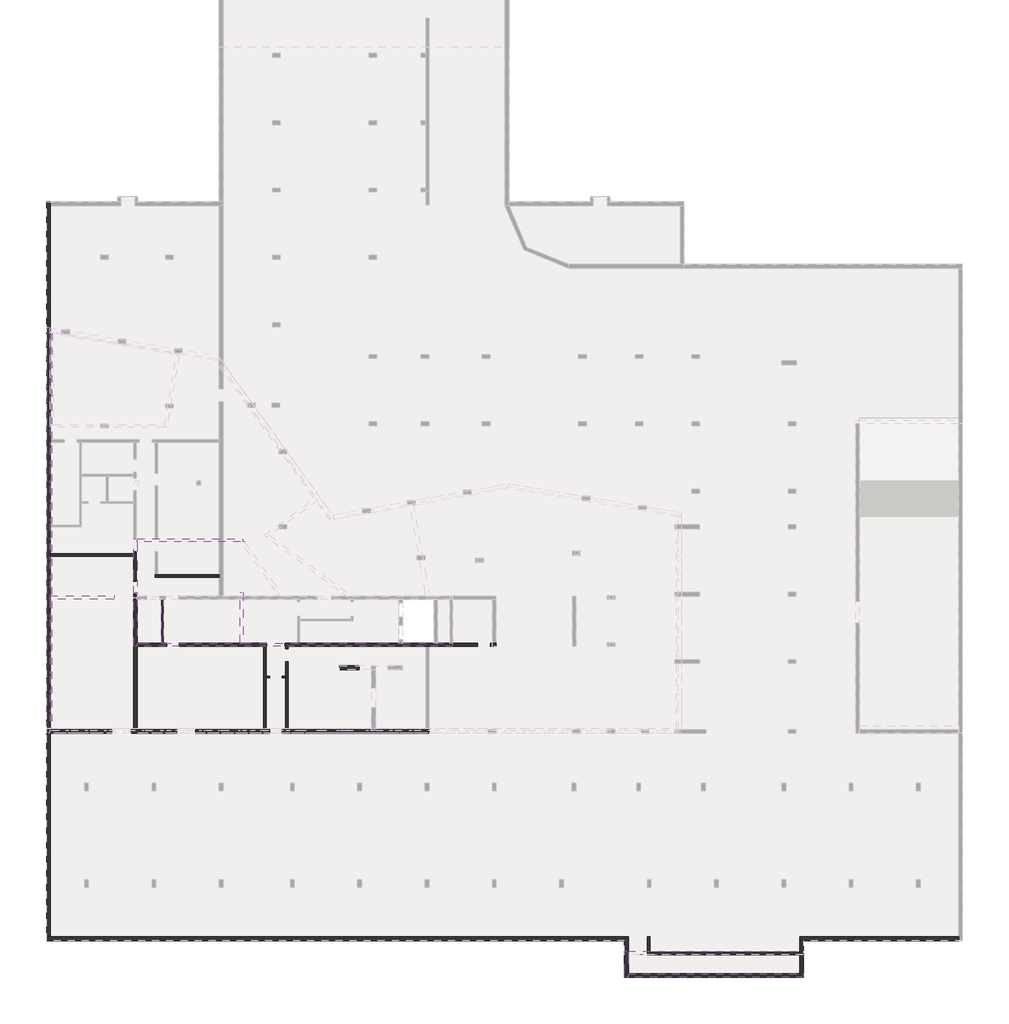
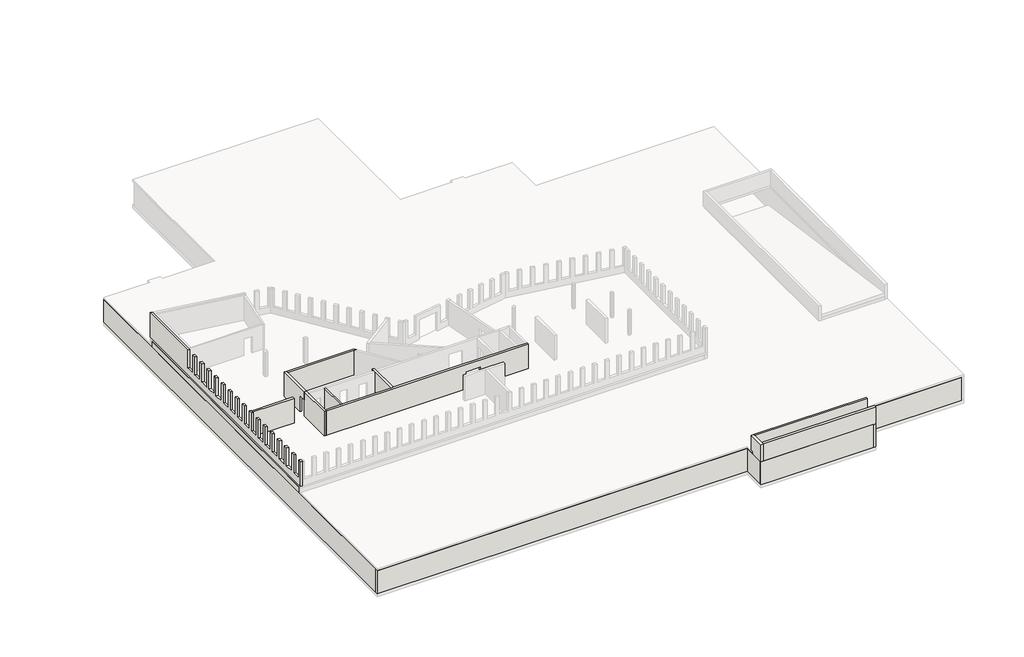
# One storey, part 1 of 4: 32 walls.
"""IFC4 building model written with IfcOpenShell, lengths in millimetres."""

from ifc_helpers import new_model, si_unit, frame, origin, place, context, project, spatial, polyline, outline, extrude, faceted_brep, element, save

model = new_model("IFC4")

# Units and contexts
model_context = context("Model", 3, world=origin())
ifc_project = project(units=[si_unit("LENGTHUNIT", "METRE", prefix="MILLI")], contexts=[model_context])

# Site, building, storey
site = spatial("IfcSite", under=ifc_project)
building = spatial("IfcBuilding", under=site)
storey = spatial("IfcBuildingStorey", under=building, Name="01_UG_OKFB_-4,20", Elevation=-4200.0)

# Walls
placement = place(None, origin())
element("IfcWall", 1, ObjectType="5dki Lochfassade 26cm C30/37", at=placement, inside=storey, context=model_context, shape_type="Brep", body=[
    faceted_brep([(130.0010047, 22777.9895381, 710.0), (130.0010047, 22777.9895381, 3060.0), (130.0010047, 22357.0124158, 3060.0), (130.0010047, 22357.0124158, 710.0), (130.0010047, 21277.0124158, 710.0), (130.0010047, 21277.0124158, 3060.0), (130.0010047, 20857.0124158, 3060.0), (130.0010047, 20857.0124158, 710.0), (130.0010047, 19777.0124158, 710.0), (130.0010047, 19777.0124158, 3060.0), (130.0010047, 19357.0124158, 3060.0), (130.0010047, 19357.0124158, 710.0), (130.0010047, 18277.0124158, 710.0), (130.0010047, 18277.0124158, 3060.0), (130.0010047, 17857.0124158, 3060.0), (130.0010047, 17857.0124158, 710.0), (130.0010047, 16777.0124158, 710.0), (130.0010047, 16777.0124158, 3060.0), (130.0010047, 16357.0124158, 3060.0), (130.0010047, 16357.0124158, 710.0), (130.0010047, 15277.0124158, 710.0), (130.0010047, 15277.0124158, 3060.0), (130.0010047, 14857.0124158, 3060.0), (130.0010047, 14857.0124158, 710.0), (130.0010047, 13777.0124158, 710.0), (130.0010047, 13777.0124158, 3060.0), (130.0010047, 13357.0124158, 3060.0), (130.0010047, 13357.0124158, 710.0), (130.0010047, 12277.0124158, 710.0), (130.0010047, 12277.0124158, 3060.0), (130.0010047, 11857.0124158, 3060.0), (130.0010047, 11857.0124158, 710.0), (130.0010047, 10777.0124158, 710.0), (130.0010047, 10777.0124158, 3060.0), (130.0010047, 10692.0124295, 3060.0), (130.0010047, 10442.0124295, 3060.0), (130.0010047, 10357.0124158, 3060.0), (130.0010047, 10357.0124158, 710.0), (130.0010047, 9277.0124158, 710.0), (130.0010047, 9277.0124158, 3060.0), (130.0010047, 8857.0124158, 3060.0), (130.0010047, 8857.0124158, 710.0), (130.0010047, 7777.0124158, 710.0), (130.0010047, 7777.0124158, 3060.0), (130.0010047, 7357.0124158, 3060.0), (130.0010047, 7357.0124158, 710.0), (130.0010047, 6277.0124158, 710.0), (130.0010047, 6277.0124158, 3060.0), (130.0010047, 5857.0124158, 3060.0), (130.0010047, 5857.0124158, 710.0), (130.0010047, 4777.0124158, 710.0), (130.0010047, 4777.0124158, 3060.0), (130.0010047, 4357.0124158, 3060.0), (130.0010047, 4357.0124158, 710.0), (130.0010047, 3277.0124158, 710.0), (130.0010047, 3277.0124158, 3060.0), (130.0010047, 2857.0124158, 3060.0), (130.0010047, 2857.0124158, 710.0), (130.0010047, 1777.0124158, 710.0), (130.0010047, 1777.0124158, 3060.0), (130.0010047, 1357.0124158, 3060.0), (130.0010047, 1357.0124158, 710.0), (130.0010047, 277.0124158, 710.0), (130.0010047, 277.0124158, 3060.0), (130.0010047, 130.000972, 3060.0), (130.0010047, -129.999028, 3060.0), (130.0010047, -129.999028, -150.0), (130.0010047, 130.000972, -150.0), (130.0010047, 10442.0124295, -150.0), (130.0010047, 10692.0124295, -150.0), (130.0010047, 31548.6978518, -150.0), (130.0010047, 31812.2980067, -150.0), (130.0010047, 31812.2980067, 3060.0), (130.0010047, 31548.6978518, 3060.0), (130.0010047, 23857.9895381, 3060.0), (130.0010047, 23857.9895381, 710.0), (-129.9989953, 22357.0124158, 3060.0), (-129.9989953, 22777.9895381, 3060.0), (-129.9989953, 22777.9895381, 710.0), (-129.9989953, 23857.9895381, 710.0), (-129.9989953, 23857.9895381, 3060.0), (-129.9989953, 31855.7150729, 3060.0), (-129.9989953, 31855.7150729, -150.0), (-129.9989953, -129.9990284, -150.0), (-129.9989953, -129.9990284, 3060.0), (-129.9989953, 277.0124158, 3060.0), (-129.9989953, 277.0124158, 710.0), (-129.9989953, 1357.0124158, 710.0), (-129.9989953, 1357.0124158, 3060.0), (-129.9989953, 1777.0124158, 3060.0), (-129.9989953, 1777.0124158, 710.0), (-129.9989953, 2857.0124158, 710.0), (-129.9989953, 2857.0124158, 3060.0), (-129.9989953, 3277.0124158, 3060.0), (-129.9989953, 3277.0124158, 710.0), (-129.9989953, 4357.0124158, 710.0), (-129.9989953, 4357.0124158, 3060.0), (-129.9989953, 4777.0124158, 3060.0), (-129.9989953, 4777.0124158, 710.0), (-129.9989953, 5857.0124158, 710.0), (-129.9989953, 5857.0124158, 3060.0), (-129.9989953, 6277.0124158, 3060.0), (-129.9989953, 6277.0124158, 710.0), (-129.9989953, 7357.0124158, 710.0), (-129.9989953, 7357.0124158, 3060.0), (-129.9989953, 7777.0124158, 3060.0), (-129.9989953, 7777.0124158, 710.0), (-129.9989953, 8857.0124158, 710.0), (-129.9989953, 8857.0124158, 3060.0), (-129.9989953, 9277.0124158, 3060.0), (-129.9989953, 9277.0124158, 710.0), (-129.9989953, 10357.0124158, 710.0), (-129.9989953, 10357.0124158, 3060.0), (-129.9989953, 10777.0124158, 3060.0), (-129.9989953, 10777.0124158, 710.0), (-129.9989953, 11857.0124158, 710.0), (-129.9989953, 11857.0124158, 3060.0), (-129.9989953, 12277.0124158, 3060.0), (-129.9989953, 12277.0124158, 710.0), (-129.9989953, 13357.0124158, 710.0), (-129.9989953, 13357.0124158, 3060.0), (-129.9989953, 13777.0124158, 3060.0), (-129.9989953, 13777.0124158, 710.0), (-129.9989953, 14857.0124158, 710.0), (-129.9989953, 14857.0124158, 3060.0), (-129.9989953, 15277.0124158, 3060.0), (-129.9989953, 15277.0124158, 710.0), (-129.9989953, 16357.0124158, 710.0), (-129.9989953, 16357.0124158, 3060.0), (-129.9989953, 16777.0124158, 3060.0), (-129.9989953, 16777.0124158, 710.0), (-129.9989953, 17857.0124158, 710.0), (-129.9989953, 17857.0124158, 3060.0), (-129.9989953, 18277.0124158, 3060.0), (-129.9989953, 18277.0124158, 710.0), (-129.9989953, 19357.0124158, 710.0), (-129.9989953, 19357.0124158, 3060.0), (-129.9989953, 19777.0124158, 3060.0), (-129.9989953, 19777.0124158, 710.0), (-129.9989953, 20857.0124158, 710.0), (-129.9989953, 20857.0124158, 3060.0), (-129.9989953, 21277.0124158, 3060.0), (-129.9989953, 21277.0124158, 710.0), (-129.9989953, 22357.0124158, 710.0)], [[[0, 1, 2, 3, 4, 5, 6, 7, 8, 9, 10, 11, 12, 13, 14, 15, 16, 17, 18, 19, 20, 21, 22, 23, 24, 25, 26, 27, 28, 29, 30, 31, 32, 33, 34, 35, 36, 37, 38, 39, 40, 41, 42, 43, 44, 45, 46, 47, 48, 49, 50, 51, 52, 53, 54, 55, 56, 57, 58, 59, 60, 61, 62, 63, 64, 65, 66, 67, 68, 69, 70, 71, 72, 73, 74, 75]], [[76, 77, 78, 79, 80, 81, 82, 83, 84, 85, 86, 87, 88, 89, 90, 91, 92, 93, 94, 95, 96, 97, 98, 99, 100, 101, 102, 103, 104, 105, 106, 107, 108, 109, 110, 111, 112, 113, 114, 115, 116, 117, 118, 119, 120, 121, 122, 123, 124, 125, 126, 127, 128, 129, 130, 131, 132, 133, 134, 135, 136, 137, 138, 139, 140, 141, 142, 143]], [[71, 70, 69, 68, 67, 66, 83, 82]], [[84, 65, 64, 63, 85]], [[60, 59, 89, 88]], [[56, 55, 93, 92]], [[52, 51, 97, 96]], [[48, 47, 101, 100]], [[44, 43, 105, 104]], [[40, 39, 109, 108]], [[36, 35, 34, 33, 113, 112]], [[30, 29, 117, 116]], [[26, 25, 121, 120]], [[22, 21, 125, 124]], [[18, 17, 129, 128]], [[14, 13, 133, 132]], [[10, 9, 137, 136]], [[6, 5, 141, 140]], [[2, 1, 77, 76]], [[74, 73, 72, 81, 80]], [[72, 71, 82, 81]], [[66, 65, 84, 83]], [[87, 61, 60, 88]], [[62, 86, 85, 63]], [[61, 87, 86, 62]], [[92, 91, 57, 56]], [[90, 89, 59, 58]], [[91, 90, 58, 57]], [[96, 95, 53, 52]], [[94, 93, 55, 54]], [[95, 94, 54, 53]], [[100, 99, 49, 48]], [[98, 97, 51, 50]], [[99, 98, 50, 49]], [[104, 103, 45, 44]], [[102, 101, 47, 46]], [[103, 102, 46, 45]], [[108, 107, 41, 40]], [[106, 105, 43, 42]], [[107, 106, 42, 41]], [[112, 111, 37, 36]], [[110, 109, 39, 38]], [[111, 110, 38, 37]], [[116, 115, 31, 30]], [[114, 113, 33, 32]], [[115, 114, 32, 31]], [[120, 119, 27, 26]], [[118, 117, 29, 28]], [[119, 118, 28, 27]], [[124, 123, 23, 22]], [[122, 121, 25, 24]], [[123, 122, 24, 23]], [[128, 127, 19, 18]], [[126, 125, 21, 20]], [[127, 126, 20, 19]], [[132, 131, 15, 14]], [[130, 129, 17, 16]], [[131, 130, 16, 15]], [[136, 135, 11, 10]], [[134, 133, 13, 12]], [[135, 134, 12, 11]], [[140, 139, 7, 6]], [[138, 137, 9, 8]], [[139, 138, 8, 7]], [[76, 143, 3, 2]], [[142, 141, 5, 4]], [[143, 142, 4, 3]], [[80, 79, 75, 74]], [[78, 77, 1, 0]], [[79, 78, 0, 75]]]),
])
element("IfcWall", 2, ObjectType="5dki STB-Wand Kern 25cm C30/37", at=placement, inside=storey, context=model_context, shape_type="Brep", body=[
    faceted_brep([(6989.9999766, 15192.0124447, 3060.0), (6989.9999766, 14942.0124447, 3060.0), (6989.9999766, 10947.0136187, 3060.0), (6989.9999766, 10947.0136187, 1985.0), (6989.9999766, 11957.013616, 1985.0), (6989.9999766, 11957.013616, -150.0), (6989.9999766, 14942.0124447, -150.0), (6989.9999766, 15192.0124447, -150.0), (6739.9999766, 10947.0136187, 3060.0), (6739.9999766, 15192.0124447, 3060.0), (6739.9999766, 15192.0124447, -150.0), (6739.9999766, 11957.013616, -150.0), (6739.9999766, 11957.013616, 1985.0), (6739.9999766, 10947.0136187, 1985.0)], [[[0, 1, 2, 3, 4, 5, 6, 7]], [[8, 9, 10, 11, 12, 13]], [[10, 7, 6, 5, 11]], [[2, 1, 0, 9, 8]], [[2, 8, 13, 3]], [[0, 7, 10, 9]], [[4, 12, 11, 5]], [[12, 4, 3, 13]]]),
])
element("IfcWall", 3, ObjectType="5dki STB-Wand Kern 25cm C30/37", at=placement, inside=storey, context=model_context, shape_type="Brep", body=[
    faceted_brep([(6989.9999766, 14942.0124447, -150.0), (15141.8279932, 14942.0124447, -150.0), (15449.8792779, 14942.0124447, -150.0), (15449.8792779, 14942.0124447, 3060.0), (15141.8279932, 14942.0124447, 3060.0), (6989.9999766, 14942.0124447, 3060.0), (6989.9999766, 15192.0124447, -150.0), (6989.9999766, 15192.0124447, 3060.0), (15269.8915173, 15192.0124447, 3060.0), (15269.8915173, 15192.0124447, -150.0)], [[[0, 1, 2, 3, 4, 5]], [[6, 7, 8, 9]], [[2, 1, 0, 6, 9]], [[5, 4, 3, 8, 7]], [[0, 5, 7, 6]], [[3, 2, 9, 8]]]),
])
element("IfcWall", 4, ObjectType="5dki STB-Wand Kern 25cm C30/37", at=placement, inside=storey, context=model_context, shape_type="Brep", body=[
    faceted_brep([(6739.9995723, 10947.0136187, -150.0), (6739.9995723, 6740.0000204, -150.0), (6739.9995723, 6740.0000204, 3060.0), (6739.9995723, 10947.0136187, 3060.0), (6739.9995723, 10947.0136187, 1985.0), (6989.9995723, 10947.0136187, -150.0), (6989.9995723, 10947.0136187, 1985.0), (6989.9995723, 10947.0136187, 3060.0), (6989.9995723, 10662.0127052, 3060.0), (6989.9995723, 10442.0127052, 3060.0), (6989.9995723, 6960.0000208, 3060.0), (6989.9995723, 6740.0000208, 3060.0), (6989.9995723, 6740.0000208, -150.0), (6989.9995723, 6960.0000208, -150.0), (6989.9995723, 10442.0127052, -150.0), (6989.9995723, 10662.0127052, -150.0)], [[[0, 1, 2, 3, 4]], [[5, 6, 7, 8, 9, 10, 11, 12, 13, 14, 15]], [[1, 0, 5, 15, 14, 13, 12]], [[3, 2, 11, 10, 9, 8, 7]], [[0, 4, 3, 7, 6, 5]], [[2, 1, 12, 11]]]),
])
element("IfcWall", 5, ObjectType="5dki STB-Wand Kern 22cm C30/37", at=placement, inside=storey, context=model_context, shape_type="Brep", body=[
    faceted_brep([(31841.999935, 6740.0000516, 3060.0), (6989.9995723, 6740.0000208, 3060.0), (6989.9995723, 6740.0000208, -150.0), (24166.9999591, 6740.0000421, -150.0), (24166.999888, 6740.0000421, 2110.0), (25926.9999591, 6740.0000443, 2110.0), (25927.000338, 6740.0000443, -150.0), (31841.999935, 6740.0000516, -150.0), (6989.9995723, 6960.0000208, 3060.0), (8916.9999886, 6960.0000232, 3060.0), (9066.9999886, 6960.0000233, 3060.0), (15117.0008797, 6960.0000309, 3060.0), (15367.0008797, 6960.0000312, 3060.0), (27641.9999886, 6960.0000464, 3060.0), (27891.9999886, 6960.0000467, 3060.0), (30391.9999891, 6960.0000498, 3060.0), (30641.9999891, 6960.0000501, 3060.0), (31641.9999382, 6960.0000514, 3060.0), (31841.9999382, 6960.0000516, 3060.0), (31841.9999382, 6960.0000516, -150.0), (31641.9999382, 6960.0000514, -150.0), (30641.9999891, 6960.0000501, -150.0), (30391.9999891, 6960.0000498, -150.0), (27891.9999886, 6960.0000467, -150.0), (27641.9999886, 6960.0000464, -150.0), (25926.9999588, 6960.0000443, -150.0), (25927.000338, 6960.0000443, 2110.0), (24166.9999588, 6960.0000421, 2110.0), (24166.999888, 6960.0000421, -150.0), (15367.0008797, 6960.0000312, -150.0), (15117.0008797, 6960.0000309, -150.0), (9066.9999886, 6960.0000233, -150.0), (8916.9999886, 6960.0000232, -150.0), (6989.9995723, 6960.0000208, -150.0)], [[[0, 1, 2, 3, 4, 5, 6, 7]], [[8, 9, 10, 11, 12, 13, 14, 15, 16, 17, 18, 19, 20, 21, 22, 23, 24, 25, 26, 27, 28, 29, 30, 31, 32, 33]], [[2, 33, 32, 31, 30, 29, 28, 3]], [[19, 7, 6, 25, 24, 23, 22, 21, 20]], [[1, 0, 18, 17, 16, 15, 14, 13, 12, 11, 10, 9, 8]], [[2, 1, 8, 33]], [[0, 7, 19, 18]], [[5, 26, 25, 6]], [[26, 5, 4, 27]], [[27, 4, 3, 28]]]),
])
element("IfcWall", 6, ObjectType="5dki STB-Wand Kern 25cm C30/37", at=placement, inside=storey, context=model_context, shape_type="SweptSolid", body=[
    extrude(outline(polyline([(15117.0008797, 6960.0000309), (15117.0008797, 10990.000031), (15367.0008797, 10990.000031), (15367.0008797, 6960.0000312), (15117.0008797, 6960.0000309)])), frame((0.0, 0.0, -150.0), z_axis=(0.0, 0.0, 1.0), x_axis=(1.0, 0.0, 0.0)), (0.0, 0.0, 1.0), 3210.0),
])
element("IfcWall", 7, ObjectType="5dki STB-Wand Kern 15cm C30/37", at=placement, inside=storey, context=model_context, shape_type="SweptSolid", body=[
    extrude(outline(polyline([(8916.9999886, 6960.0000232), (8916.9999886, 10442.0127087), (9066.9999886, 10442.0127089), (9066.9999886, 6960.0000233), (8916.9999886, 6960.0000232)])), frame((0.0, 0.0, -150.0), z_axis=(0.0, 0.0, 1.0), x_axis=(1.0, 0.0, 0.0)), (0.0, 0.0, 1.0), 3210.0),
])
element("IfcWall", 8, ObjectType="5dki STB-Wand Kern 22cm C30/37", at=placement, inside=storey, context=model_context, shape_type="Brep", body=[
    faceted_brep([(35269.999309, 6740.0016809, -1200.0), (29969.9992095, 6740.0014024, -1200.0), (29769.9992095, 6740.0013919, -1200.0), (18876.9410665, 6740.0008196, -1200.0), (18676.9410665, 6740.0008091, -1200.0), (17176.9410653, 6740.0007303, -1200.0), (16976.9410653, 6740.0007198, -1200.0), (6990.0006232, 6740.0001951, -1200.0), (6740.000624, 6740.0001819, -1200.0), (6740.000624, 6740.0001819, -4200.0), (6990.0006232, 6740.0001951, -4200.0), (9318.2481994, 6740.0003174, -4200.0), (9318.2482224, 6740.0003174, -2065.0), (10328.2481994, 6740.0003705, -2065.0), (10328.248215, 6740.0003705, -4200.0), (16976.9410653, 6740.0007198, -4200.0), (17176.9410653, 6740.0007303, -4200.0), (17186.9410653, 6740.0007308, -4200.0), (17186.9410832, 6740.0007308, -2065.0), (18666.9410653, 6740.0008086, -2065.0), (18666.9410837, 6740.0008086, -4200.0), (18676.9410665, 6740.0008091, -4200.0), (18876.9410665, 6740.0008196, -4200.0), (29769.9992095, 6740.0013919, -4200.0), (29969.9992095, 6740.0014024, -4200.0), (33806.9997689, 6740.001604, -4200.0), (33806.9997878, 6740.001604, -2065.0), (34816.9997689, 6740.0016571, -2065.0), (34816.9998011, 6740.0016571, -4200.0), (35269.999309, 6740.0016809, -4200.0), (6740.0006072, 6960.0001819, -1200.0), (6990.0006072, 6960.0001951, -1200.0), (8916.9991145, 6960.0002963, -1200.0), (9066.9991145, 6960.0003042, -1200.0), (19626.9996762, 6960.000859, -1200.0), (19776.9996762, 6960.0008669, -1200.0), (27642.0002944, 6960.0012801, -1200.0), (27892.0002944, 6960.0012933, -1200.0), (30391.9991141, 6960.0014246, -1200.0), (30641.9991141, 6960.0014377, -1200.0), (31641.9991143, 6960.0014903, -1200.0), (31841.9991143, 6960.0015008, -1200.0), (34969.9993085, 6960.0016651, -1200.0), (35269.9993085, 6960.0016809, -1200.0), (35269.9993085, 6960.0016809, -4200.0), (34969.9993085, 6960.0016651, -4200.0), (34816.9997573, 6960.0016571, -4200.0), (34816.9997599, 6960.0016571, -2065.0), (33806.9997573, 6960.001604, -2065.0), (33806.9997466, 6960.001604, -4200.0), (31841.9991143, 6960.0015008, -4200.0), (31641.9991143, 6960.0014903, -4200.0), (30641.9991141, 6960.0014377, -4200.0), (30391.9991141, 6960.0014246, -4200.0), (27892.0002944, 6960.0012933, -4200.0), (27642.0002944, 6960.0012801, -4200.0), (19776.9996762, 6960.0008669, -4200.0), (19626.9996762, 6960.000859, -4200.0), (18666.9410538, 6960.0008086, -4200.0), (18666.9410424, 6960.0008086, -2065.0), (17186.9410538, 6960.0007308, -2065.0), (17186.941042, 6960.0007308, -4200.0), (10328.2481878, 6960.0003705, -4200.0), (10328.2481738, 6960.0003705, -2065.0), (9318.2481878, 6960.0003174, -2065.0), (9318.2481812, 6960.0003174, -4200.0), (9066.9991145, 6960.0003042, -4200.0), (8916.9991145, 6960.0002963, -4200.0), (6990.0006072, 6960.0001951, -4200.0), (6740.0006072, 6960.0001819, -4200.0)], [[[0, 1, 2, 3, 4, 5, 6, 7, 8, 9, 10, 11, 12, 13, 14, 15, 16, 17, 18, 19, 20, 21, 22, 23, 24, 25, 26, 27, 28, 29]], [[30, 31, 32, 33, 34, 35, 36, 37, 38, 39, 40, 41, 42, 43, 44, 45, 46, 47, 48, 49, 50, 51, 52, 53, 54, 55, 56, 57, 58, 59, 60, 61, 62, 63, 64, 65, 66, 67, 68, 69]], [[44, 29, 28, 46, 45]], [[9, 69, 68, 67, 66, 65, 11, 10]], [[49, 25, 24, 23, 22, 21, 20, 58, 57, 56, 55, 54, 53, 52, 51, 50]], [[14, 62, 61, 17, 16, 15]], [[8, 7, 6, 5, 4, 3, 2, 1, 0, 43, 42, 41, 40, 39, 38, 37, 36, 35, 34, 33, 32, 31, 30]], [[0, 29, 44, 43]], [[9, 8, 30, 69]], [[27, 47, 46, 28]], [[47, 27, 26, 48]], [[48, 26, 25, 49]], [[64, 12, 11, 65]], [[12, 64, 63, 13]], [[13, 63, 62, 14]], [[60, 18, 17, 61]], [[18, 60, 59, 19]], [[19, 59, 58, 20]]]),
])
element("IfcWall", 9, ObjectType="5dki STB-Wand Kern 25cm C30/37", at=placement, inside=storey, context=model_context, shape_type="SweptSolid", body=[
    extrude(outline(polyline([(6740.0006072, 6960.0001819), (6740.0003427, 10442.0129553), (6990.0003427, 10442.0129495), (6990.0006072, 6960.0001951), (6740.0006072, 6960.0001819)])), frame((0.0, 0.0, -4200.0), z_axis=(0.0, 0.0, 1.0), x_axis=(1.0, 0.0, 0.0)), (0.0, 0.0, 1.0), 3000.0),
])
element("IfcWall", 10, ObjectType="5dki STB-Wand Kern 15cm C30/37", at=placement, inside=storey, context=model_context, shape_type="SweptSolid", body=[
    extrude(outline(polyline([(8916.9991145, 6960.0002963), (8916.9991145, 10442.012905), (9066.9991145, 10442.0129015), (9066.9991145, 6960.0003042), (8916.9991145, 6960.0002963)])), frame((0.0, 0.0, -4200.0), z_axis=(0.0, 0.0, 1.0), x_axis=(1.0, 0.0, 0.0)), (0.0, 0.0, 1.0), 3000.0),
])
element("IfcWall", 11, ObjectType="5dki STB-Wand 30cm WU C35/45", at=placement, inside=storey, context=model_context, shape_type="Brep", body=[
    faceted_brep([(71679.9986191, -16130.0005666, -4200.0), (59176.9101139, -16130.0005666, -4200.0), (59176.9101139, -16130.0005666, -1200.0), (71679.9986191, -16130.0005666, -1200.0), (71679.9986133, -16430.0005666, -4200.0), (71679.9986133, -16430.0005666, -1200.0), (59476.9101139, -16430.0005666, -1200.0), (59176.9101139, -16430.0005666, -1200.0), (59176.9101139, -16430.0005666, -4200.0), (59476.9101139, -16430.0005666, -4200.0)], [[[0, 1, 2, 3]], [[4, 5, 6, 7, 8, 9]], [[1, 0, 4, 9, 8]], [[3, 2, 7, 6, 5]], [[0, 3, 5, 4]], [[2, 1, 8, 7]]]),
])
element("IfcWall", 12, ObjectType="5dki STB-Wand 30cm WU C35/45", at=placement, inside=storey, context=model_context, shape_type="Brep", body=[
    faceted_brep([(59176.9101139, -16430.0005666, -4200.0), (59176.9101139, -17332.4969559, -4200.0), (59176.9101139, -17532.4969604, -4200.0), (59176.9101139, -19032.4966002, -4200.0), (59176.9101139, -19332.4966002, -4200.0), (59176.9101139, -19332.4966002, -1200.0), (59176.9101139, -19032.4966002, -1200.0), (59176.9101139, -17532.4969604, -1200.0), (59176.9101139, -17332.4969559, -1200.0), (59176.9101139, -16430.0005666, -1200.0), (59476.9101139, -16430.0005666, -4200.0), (59476.9101139, -16430.0005666, -1200.0), (59476.9101139, -19332.4966002, -1200.0), (59476.9101139, -19332.4966002, -4200.0)], [[[0, 1, 2, 3, 4, 5, 6, 7, 8, 9]], [[10, 11, 12, 13]], [[4, 3, 2, 1, 0, 10, 13]], [[9, 8, 7, 6, 5, 12, 11]], [[0, 9, 11, 10]], [[5, 4, 13, 12]]]),
])
element("IfcWall", 13, ObjectType="5dki STB-Wand 30cm WU C35/45", at=placement, inside=storey, context=model_context, shape_type="Brep", body=[
    faceted_brep([(59176.9101139, -19032.4966002, -4200.0), (45670.0209209, -19032.4966002, -4200.0), (45370.0209209, -19032.4966002, -4200.0), (45370.0209209, -19032.4966002, -1200.0), (45670.0209209, -19032.4966002, -1200.0), (59176.9101139, -19032.4966002, -1200.0), (59176.9101139, -19332.4966002, -4200.0), (59176.9101139, -19332.4966002, -1200.0), (45370.0209209, -19332.4966002, -1200.0), (45370.0209209, -19332.4966002, -4200.0)], [[[0, 1, 2, 3, 4, 5]], [[6, 7, 8, 9]], [[2, 1, 0, 6, 9]], [[5, 4, 3, 8, 7]], [[0, 5, 7, 6]], [[3, 2, 9, 8]]]),
])
element("IfcWall", 14, ObjectType="5dki STB-Wand 30cm WU C35/45", at=placement, inside=storey, context=model_context, shape_type="Brep", body=[
    faceted_brep([(45670.0209209, -19032.4966002, -4200.0), (45670.0209209, -16129.9998873, -4200.0), (45670.0209209, -16129.9998873, -1200.0), (45670.0209209, -19032.4966002, -1200.0), (45370.0209209, -19032.4966002, -4200.0), (45370.0209209, -19032.4966002, -1200.0), (45370.0209209, -16429.9998873, -1200.0), (45370.0209209, -16129.9998873, -1200.0), (45370.0209209, -16129.9998873, -4200.0), (45370.0209209, -16429.9998873, -4200.0)], [[[0, 1, 2, 3]], [[4, 5, 6, 7, 8, 9]], [[1, 0, 4, 9, 8]], [[3, 2, 7, 6, 5]], [[0, 3, 5, 4]], [[2, 1, 8, 7]]]),
])
element("IfcWall", 15, ObjectType="5dki STB-Wand 30cm WU C35/45", at=placement, inside=storey, context=model_context, shape_type="Brep", body=[
    faceted_brep([(45370.0209209, -16129.9998873, -4200.0), (169.9998112, -16129.9998873, -4200.0), (-130.0001888, -16129.9998873, -4200.0), (-130.0001888, -16129.9998873, -1200.0), (169.9998112, -16129.9998873, -1200.0), (45370.0209209, -16129.9998873, -1200.0), (45370.0209209, -16429.9998873, -4200.0), (45370.0209209, -16429.9998873, -1200.0), (-130.0001888, -16429.9998873, -1200.0), (-130.0001888, -16429.9998873, -4200.0)], [[[0, 1, 2, 3, 4, 5]], [[6, 7, 8, 9]], [[2, 1, 0, 6, 9]], [[5, 4, 3, 8, 7]], [[0, 5, 7, 6]], [[3, 2, 9, 8]]]),
])
element("IfcWall", 16, ObjectType="5dki STB-Wand 30cm WU C35/45", at=placement, inside=storey, context=model_context, shape_type="Brep", body=[
    faceted_brep([(169.9998112, -16129.9998873, -4200.0), (169.9998112, -129.9999484, -4200.0), (169.9998112, 170.0000516, -4200.0), (169.9998112, 13818.6536257, -4200.0), (169.9998112, 14018.6536257, -4200.0), (169.9998112, 22769.9814538, -4200.0), (169.9998112, 22969.9814538, -4200.0), (169.9998112, 41417.0011496, -4200.0), (169.9998112, 41717.0011496, -4200.0), (169.9998112, 41717.0011496, -1200.0), (169.9998112, 41417.0011496, -1200.0), (169.9998112, 22969.9814538, -1200.0), (169.9998112, 22769.9814538, -1200.0), (169.9998112, 14018.6536257, -1200.0), (169.9998112, 13818.6536257, -1200.0), (169.9998112, 170.0000516, -1200.0), (169.9998112, -129.9999484, -1200.0), (169.9998112, -16129.9998873, -1200.0), (-130.0001888, -16129.9998873, -4200.0), (-130.0001888, -16129.9998873, -1200.0), (-130.0001888, 41717.0011496, -1200.0), (-130.0001888, 41717.0011496, -4200.0)], [[[0, 1, 2, 3, 4, 5, 6, 7, 8, 9, 10, 11, 12, 13, 14, 15, 16, 17]], [[18, 19, 20, 21]], [[8, 7, 6, 5, 4, 3, 2, 1, 0, 18, 21]], [[17, 16, 15, 14, 13, 12, 11, 10, 9, 20, 19]], [[0, 17, 19, 18]], [[9, 8, 21, 20]]]),
])
element("IfcWall", 17, ObjectType="5dki Überzug 40cm C30/37", at=placement, inside=storey, context=model_context, shape_type="Brep", body=[
    faceted_brep([(269.9998112, 270.0010491, -1200.0), (269.9998112, 31383.3810859, -1200.0), (269.9998112, 31383.3810859, -400.0), (269.9998112, 270.0010491, -400.0), (-130.0001888, 270.0010491, -1200.0), (-130.0001888, 270.0010491, -950.0), (-130.0001888, 270.0010491, -400.0), (-130.0001888, 31450.1765724, -400.0), (-130.0001888, 31450.1765724, -950.0), (-130.0001888, 31450.1765724, -1200.0)], [[[0, 1, 2, 3]], [[4, 5, 6, 7, 8, 9]], [[1, 0, 4, 9]], [[3, 2, 7, 6]], [[2, 1, 9, 8, 7]], [[0, 3, 6, 5, 4]]]),
])
element("IfcWall", 18, ObjectType="5dki STB-Wand 12,5cm C20/25", at=placement, inside=storey, context=model_context, shape_type="Brep", body=[
    faceted_brep([(18676.94108, 4233.966015, -1200.0), (17176.9410795, 4233.9660069, -1200.0), (17176.9410795, 4233.9660069, -4200.0), (17421.9417385, 4233.9660083, -4200.0), (17421.9417453, 4233.9660083, -2065.0), (18431.9417385, 4233.9660137, -2065.0), (18431.9417669, 4233.9660137, -4200.0), (18676.94108, 4233.966015, -4200.0), (17176.9410788, 4358.9660069, -1200.0), (18676.9410794, 4358.966015, -1200.0), (18676.9410794, 4358.966015, -4200.0), (18431.9417378, 4358.9660137, -4200.0), (18431.9417669, 4358.9660137, -2065.0), (17421.9417378, 4358.9660083, -2065.0), (17421.9417453, 4358.9660083, -4200.0), (17176.9410788, 4358.9660069, -4200.0)], [[[0, 1, 2, 3, 4, 5, 6, 7]], [[8, 9, 10, 11, 12, 13, 14, 15]], [[2, 15, 14, 3]], [[10, 7, 6, 11]], [[1, 0, 9, 8]], [[2, 1, 8, 15]], [[0, 7, 10, 9]], [[5, 12, 11, 6]], [[12, 5, 4, 13]], [[13, 4, 3, 14]]]),
])
element("IfcWall", 19, ObjectType="5dki STB-Wand 20cm C25/30", at=placement, inside=storey, context=model_context, shape_type="Brep", body=[
    faceted_brep([(13469.9992636, 12367.0009111, -4200.0), (8640.0000033, 12367.0009111, -4200.0), (8440.0000033, 12367.0009111, -4200.0), (8440.0000033, 12367.0009111, -1200.0), (8640.0000033, 12367.0009111, -1200.0), (13469.9992636, 12367.0009111, -1200.0), (13469.9992584, 12167.0009111, -4200.0), (13469.9992584, 12167.0009111, -1200.0), (8439.9999991, 12167.0009111, -1200.0), (8439.9999991, 12167.0009111, -4200.0)], [[[0, 1, 2, 3, 4, 5]], [[6, 7, 8, 9]], [[2, 1, 0, 6, 9]], [[5, 4, 3, 8, 7]], [[0, 5, 7, 6]], [[3, 2, 9, 8]]]),
])
element("IfcWall", 20, ObjectType="5dki STB-Wand 20cm C30/37", at=placement, inside=storey, context=model_context, shape_type="Brep", body=[
    faceted_brep([(47169.9986162, -16129.9999339, -4200.0), (47169.9986162, -17529.9576362, -4200.0), (47169.9986162, -17529.9576362, -1200.0), (47169.9986162, -16129.9999339, -1200.0), (47369.9986162, -16129.9999339, -4200.0), (47369.9986162, -16129.9999339, -1200.0), (47369.9986162, -17329.9999295, -1200.0), (47369.9986162, -17529.9999339, -1200.0), (47369.9986162, -17529.9999339, -4200.0), (47369.9986162, -17329.9999295, -4200.0)], [[[0, 1, 2, 3]], [[4, 5, 6, 7, 8, 9]], [[1, 0, 4, 9, 8]], [[3, 2, 7, 6, 5]], [[0, 3, 5, 4]], [[2, 1, 8, 7]]]),
])
element("IfcWall", 21, ObjectType="5dki STB-Wand 20cm C30/37", at=placement, inside=storey, context=model_context, shape_type="SweptSolid", body=[
    extrude(outline(polyline([(59176.9101139, -17532.4969604), (47369.9986162, -17529.9999339), (47369.9986162, -17329.9999295), (59176.9101139, -17332.4969559), (59176.9101139, -17532.4969604)])), frame((0.0, 0.0, -4200.0), z_axis=(0.0, 0.0, 1.0), x_axis=(1.0, 0.0, 0.0)), (0.0, 0.0, 1.0), 3000.0),
])
element("IfcWall", 22, ObjectType="5dki STB-Wand 20cm C40/50", at=placement, inside=storey, context=model_context, shape_type="Brep", body=[
    faceted_brep([(17176.9411026, 170.0000516, -4200.0), (17176.9410795, 4233.9660069, -4200.0), (17176.9410788, 4358.9660069, -4200.0), (17176.9410653, 6740.0007303, -4200.0), (17176.9410653, 6740.0007303, -1200.0), (17176.9410788, 4358.9660069, -1200.0), (17176.9410795, 4233.9660069, -1200.0), (17176.9411026, 170.0000516, -1200.0), (16976.9411026, 170.0000516, -4200.0), (16976.9411026, 170.0000516, -1200.0), (16976.9410653, 6740.0007198, -1200.0), (16976.9410653, 6740.0007198, -4200.0)], [[[0, 1, 2, 3, 4, 5, 6, 7]], [[8, 9, 10, 11]], [[3, 2, 1, 0, 8, 11]], [[7, 6, 5, 4, 10, 9]], [[4, 3, 11, 10]], [[0, 7, 9, 8]]]),
])
element("IfcWall", 23, ObjectType="5dki STB-Wand 20cm C40/50", at=placement, inside=storey, context=model_context, shape_type="Brep", body=[
    faceted_brep([(18876.9410665, 6740.0008196, -1200.0), (18876.941102, 170.0000516, -1200.0), (18876.941102, 170.0000516, -4200.0), (18876.9410731, 5519.0104508, -4200.0), (18876.9410731, 5519.0104508, -2065.0), (18876.9410676, 6529.0104508, -2065.0), (18876.9410676, 6529.0104508, -4200.0), (18876.9410665, 6740.0008196, -4200.0), (18676.941102, 170.0000516, -1200.0), (18676.94108, 4233.966015, -1200.0), (18676.9410794, 4358.966015, -1200.0), (18676.9410665, 6740.0008091, -1200.0), (18676.9410665, 6740.0008091, -4200.0), (18676.9410676, 6529.0104497, -4200.0), (18676.9410676, 6529.0104497, -2065.0), (18676.9410731, 5519.0104497, -2065.0), (18676.9410731, 5519.0104497, -4200.0), (18676.9410794, 4358.966015, -4200.0), (18676.94108, 4233.966015, -4200.0), (18676.941102, 170.0000516, -4200.0)], [[[0, 1, 2, 3, 4, 5, 6, 7]], [[8, 9, 10, 11, 12, 13, 14, 15, 16, 17, 18, 19]], [[2, 19, 18, 17, 16, 3]], [[12, 7, 6, 13]], [[1, 0, 11, 10, 9, 8]], [[0, 7, 12, 11]], [[2, 1, 8, 19]], [[15, 4, 3, 16]], [[4, 15, 14, 5]], [[5, 14, 13, 6]]]),
])
element("IfcWall", 24, ObjectType="5dki STB-Wand 20cm C40/50", at=placement, inside=storey, context=model_context, shape_type="SweptSolid", body=[
    extrude(outline(polyline([(6739.9999987, 13818.6536257), (169.9998112, 13818.6536257), (169.9998112, 14018.6536257), (6740.0000008, 14018.6536257), (6739.9999987, 13818.6536257)])), frame((0.0, 0.0, -4200.0), z_axis=(0.0, 0.0, 1.0), x_axis=(1.0, 0.0, 0.0)), (0.0, 0.0, 1.0), 3000.0),
])
element("IfcWall", 25, ObjectType="5dki STB-Wand 20cm C40/50", at=placement, inside=storey, context=model_context, shape_type="Brep", body=[
    faceted_brep([(6739.9999661, 10662.0129553, -1200.0), (6739.9999987, 13818.6536257, -1200.0), (6740.0000008, 14018.6536257, -1200.0), (6740.0000023, 14168.653631, -1200.0), (6740.0000023, 14168.653631, -4200.0), (6740.0000008, 14018.6536257, -4200.0), (6739.9999987, 13818.6536257, -4200.0), (6739.9999784, 11849.505845, -4200.0), (6739.9999784, 11849.505845, -2065.0), (6739.9999679, 10839.505845, -2065.0), (6739.9999679, 10839.505845, -4200.0), (6739.9999661, 10662.0129553, -4200.0), (6940.0000023, 14168.6536289, -1200.0), (6939.9999661, 10662.0129507, -1200.0), (6939.9999661, 10662.0129507, -4200.0), (6939.9999679, 10839.5058429, -4200.0), (6939.9999679, 10839.5058429, -2065.0), (6939.9999784, 11849.5058429, -2065.0), (6939.9999784, 11849.5058429, -4200.0), (6940.0000023, 14168.6536289, -4200.0)], [[[0, 1, 2, 3, 4, 5, 6, 7, 8, 9, 10, 11]], [[12, 13, 14, 15, 16, 17, 18, 19]], [[4, 19, 18, 7, 6, 5]], [[14, 11, 10, 15]], [[3, 2, 1, 0, 13, 12]], [[4, 3, 12, 19]], [[0, 11, 14, 13]], [[17, 8, 7, 18]], [[8, 17, 16, 9]], [[9, 16, 15, 10]]]),
])
element("IfcWall", 26, ObjectType="5dki STB-Wand 25cm C30/37", at=placement, inside=storey, context=model_context, shape_type="SweptSolid", body=[
    extrude(outline(polyline([(130.0010047, 10692.0124295), (5179.9999831, 10692.0124295), (5179.9999831, 10442.0124295), (130.0010047, 10442.0124295), (130.0010047, 10692.0124295)])), frame((0.0, 0.0, -150.0), z_axis=(0.0, 0.0, 1.0), x_axis=(1.0, 0.0, 0.0)), (0.0, 0.0, 1.0), 3210.0),
])
element("IfcWall", 27, ObjectType="5dki STB-Wand 25cm C30/37", at=placement, inside=storey, context=model_context, shape_type="SweptSolid", body=[
    extrude(outline(polyline([(6990.0006232, 6740.0001951), (6990.0011205, 170.0000516), (6740.0011205, 170.0000516), (6740.0006232, 6740.0001819), (6990.0006232, 6740.0001951)])), frame((0.0, 0.0, -4200.0), z_axis=(0.0, 0.0, 1.0), x_axis=(1.0, 0.0, 0.0)), (0.0, 0.0, 1.0), 3000.0),
])
element("IfcWall", 28, ObjectType="5dki STB-Wand 25cm C30/37", at=placement, inside=storey, context=model_context, shape_type="SweptSolid", body=[
    extrude(outline(polyline([(59476.6666693, -17532.5603554), (45670.0206212, -17529.6404081), (45670.0206747, -17279.6404025), (59476.7195415, -17282.560361), (59476.6666693, -17532.5603554)])), frame((0.0, 0.0, -950.0), z_axis=(0.0, 0.0, 1.0), x_axis=(1.0, 0.0, 0.0)), (0.0, 0.0, 1.0), 1950.0),
])
element("IfcWall", 29, ObjectType="5dki STB-Wand 30cm C30/37", at=placement, inside=storey, context=model_context, shape_type="Brep", body=[
    faceted_brep([(29969.9990344, -129.9999484, -1200.0), (169.9998112, -129.9999484, -1200.0), (169.9998112, -129.9999484, -4200.0), (5009.9990394, -129.9999484, -4200.0), (5009.9990394, -129.9999484, -1940.0), (6519.9990394, -129.9999484, -1940.0), (6519.9990394, -129.9999484, -4200.0), (10108.8783928, -129.9999484, -4200.0), (10108.8783928, -129.9999484, -1940.0), (11618.8783928, -129.9999484, -1940.0), (11618.8783928, -129.9999484, -4200.0), (17421.9410854, -129.9999484, -4200.0), (17421.9410854, -129.9999484, -2065.0), (18431.9410854, -129.9999484, -2065.0), (18431.9410854, -129.9999484, -4200.0), (29969.9990344, -129.9999484, -4200.0), (169.9998112, 170.0000516, -1200.0), (6740.0011205, 170.0000516, -1200.0), (6990.0011205, 170.0000516, -1200.0), (16976.9411026, 170.0000516, -1200.0), (17176.9411026, 170.0000516, -1200.0), (18676.941102, 170.0000516, -1200.0), (18876.941102, 170.0000516, -1200.0), (25467.0001225, 170.0000516, -1200.0), (25767.0001225, 170.0000516, -1200.0), (29769.9990421, 170.0000516, -1200.0), (29969.9990421, 170.0000516, -1200.0), (29969.9990421, 170.0000516, -4200.0), (29769.9990421, 170.0000516, -4200.0), (25767.0001225, 170.0000516, -4200.0), (25467.0001225, 170.0000516, -4200.0), (18876.941102, 170.0000516, -4200.0), (18676.941102, 170.0000516, -4200.0), (18431.9410854, 170.0000516, -4200.0), (18431.9410854, 170.0000516, -2065.0), (17421.9410854, 170.0000516, -2065.0), (17421.9410854, 170.0000516, -4200.0), (17176.9411026, 170.0000516, -4200.0), (16976.9411026, 170.0000516, -4200.0), (11618.8783928, 170.0000516, -4200.0), (11618.8783928, 170.0000516, -1940.0), (10108.8783928, 170.0000516, -1940.0), (10108.8783928, 170.0000516, -4200.0), (6990.0011205, 170.0000516, -4200.0), (6740.0011205, 170.0000516, -4200.0), (6519.9990394, 170.0000516, -4200.0), (6519.9990394, 170.0000516, -1940.0), (5009.9990394, 170.0000516, -1940.0), (5009.9990394, 170.0000516, -4200.0), (169.9998112, 170.0000516, -4200.0)], [[[0, 1, 2, 3, 4, 5, 6, 7, 8, 9, 10, 11, 12, 13, 14, 15]], [[16, 17, 18, 19, 20, 21, 22, 23, 24, 25, 26, 27, 28, 29, 30, 31, 32, 33, 34, 35, 36, 37, 38, 39, 40, 41, 42, 43, 44, 45, 46, 47, 48, 49]], [[27, 15, 14, 33, 32, 31, 30, 29, 28]], [[2, 49, 48, 3]], [[6, 45, 44, 43, 42, 7]], [[10, 39, 38, 37, 36, 11]], [[1, 0, 26, 25, 24, 23, 22, 21, 20, 19, 18, 17, 16]], [[0, 15, 27, 26]], [[2, 1, 16, 49]], [[5, 46, 45, 6]], [[46, 5, 4, 47]], [[47, 4, 3, 48]], [[9, 40, 39, 10]], [[40, 9, 8, 41]], [[41, 8, 7, 42]], [[13, 34, 33, 14]], [[34, 13, 12, 35]], [[35, 12, 11, 36]]]),
])
element("IfcWall", 30, ObjectType="5dki STB-Wand 30cm C30/37", at=placement, inside=storey, context=model_context, shape_type="SweptSolid", body=[
    extrude(outline(polyline([(22936.4907985, 5180.0007355), (24467.0002549, 5180.0006968), (24467.0002474, 4880.0006968), (22936.4907909, 4880.0007355), (22936.4907985, 5180.0007355)])), frame((0.0, 0.0, -4200.0), z_axis=(0.0, 0.0, 1.0), x_axis=(1.0, 0.0, 0.0)), (0.0, 0.0, 1.0), 3000.0),
])
element("IfcWall", 31, ObjectType="5dki STB-Wand 30cm C30/37", at=placement, inside=storey, context=model_context, shape_type="Brep", body=[
    faceted_brep([(45670.0202351, -19332.4966536, -1200.0), (45670.0202994, -19032.4966536, -1200.0), (45670.0206206, -17532.5573989, -1200.0), (45670.0206206, -17532.5573989, -950.0), (45670.0206212, -17529.6404081, -950.0), (45670.0206747, -17279.6404025, -950.0), (45670.0206747, -17279.6404025, 1000.0), (45670.0206212, -17529.6404081, 1000.0), (45670.0202994, -19032.4966536, 1000.0), (45670.0202351, -19332.4966536, 1000.0), (45370.0202351, -19332.4966547, -1200.0), (45370.0202351, -19332.4966547, 1000.0), (45370.0206747, -17279.5769559, 1000.0), (45370.0206747, -17279.5769559, -950.0), (45370.0206206, -17532.5573346, -950.0), (45370.0206206, -17532.5573346, -1200.0)], [[[0, 1, 2, 3, 4, 5, 6, 7, 8, 9]], [[10, 11, 12, 13, 14, 15]], [[6, 5, 13, 12]], [[0, 9, 11, 10]], [[2, 1, 0, 10, 15]], [[9, 8, 7, 6, 12, 11]], [[3, 2, 15, 14]], [[5, 4, 3, 14, 13]]]),
])
element("IfcWall", 32, ObjectType="5dki STB-Wand 30cm C30/37", at=placement, inside=storey, context=model_context, shape_type="SweptSolid", body=[
    extrude(outline(polyline([(59476.9100357, -19332.4966002), (45670.0202351, -19332.4966536), (45670.0202994, -19032.4966536), (59476.9100345, -19032.4966002), (59476.9100357, -19332.4966002)])), frame((0.0, 0.0, -1200.0), z_axis=(0.0, 0.0, 1.0), x_axis=(1.0, 0.0, 0.0)), (0.0, 0.0, 1.0), 2200.0),
])

save(model, "model.ifc")

# Revit data of these elements
# Type "5dki Lochfassade 26cm C30/37"
#   Type Comments = ""
#   Description = ""
#   cpiComponentType = "Wall"
#   cpiFitMatchKey = "5D-KI-STB-OB-W-LF"
#   5d Materialgüte = "C35/45"
#   Filter Tragend / Nichttragend = yes
#   5dki WU = no
#   Layers, outside or top first: 0.260 m "5d Beton - Stahlbeton" (function 1)
# Type "5dki STB-Wand Kern 25cm C30/37"
#   Type Comments = ""
#   Description = ""
#   cpiComponentType = "Wall"
#   cpiFitMatchKey = "5D-KI-STB-OB-W-K"
#   5d Materialgüte = "C30/37"
#   Filter Tragend / Nichttragend = yes
#   5dki WU = no
#   Layers, outside or top first: 0.250 m "5d Beton - Stahlbeton" (function 1)
# Type "5dki STB-Wand Kern 22cm C30/37"
#   Type Comments = ""
#   Description = ""
#   cpiComponentType = "Wall"
#   cpiFitMatchKey = "5D-KI-STB-OB-W-K"
#   5d Materialgüte = "C30/37"
#   Filter Tragend / Nichttragend = yes
#   5dki WU = no
#   Layers, outside or top first: 0.220 m "5d Beton - Stahlbeton" (function 1)
# Type "5dki STB-Wand Kern 15cm C30/37"
#   Type Comments = ""
#   Description = ""
#   cpiComponentType = "Wall"
#   cpiFitMatchKey = "5D-KI-STB-OB-W-K"
#   5d Materialgüte = "C30/37"
#   Filter Tragend / Nichttragend = yes
#   5dki WU = no
#   Layers, outside or top first: 0.150 m "5d Beton - Stahlbeton" (function 1)
# Type "5dki STB-Wand 30cm WU C35/45"
#   Type Comments = ""
#   Description = ""
#   cpiComponentType = "Wall"
#   cpiFitMatchKey = "5D-KI-STB-OB-W"
#   5d Materialgüte = "C35/45"
#   Filter Tragend / Nichttragend = yes
#   5dki WU = yes
#   Layers, outside or top first: 0.300 m "5d Beton - Stahlbeton WU" (function 1)
# Type "5dki Überzug 40cm C30/37"
#   Type Comments = ""
#   Description = ""
#   cpiComponentType = "Beam"
#   cpiFitMatchKey = "5D-KI-STB-OB-TR-UEZ"
#   5d Materialgüte = "C30/37"
#   Filter Tragend / Nichttragend = yes
#   Layers, outside or top first: 0.400 m "5d Beton - Stahlbeton" (function 1)
# Type "5dki STB-Wand 12,5cm C20/25"
#   Type Comments = ""
#   Description = ""
#   cpiComponentType = "Wall"
#   cpiFitMatchKey = "5D-KI-STB-OB-W"
#   5d Materialgüte = "C20/25"
#   Filter Tragend / Nichttragend = yes
#   5dki WU = no
#   Layers, outside or top first: 0.125 m "5d Beton - Stahlbeton" (function 1)
# Type "5dki STB-Wand 20cm C25/30"
#   Type Comments = ""
#   Description = ""
#   cpiComponentType = "Wall"
#   cpiFitMatchKey = "5D-KI-STB-OB-W"
#   5d Materialgüte = "C25/30"
#   Filter Tragend / Nichttragend = yes
#   5dki WU = no
#   Layers, outside or top first: 0.200 m "5d Beton - Stahlbeton" (function 1)
# Type "5dki STB-Wand 20cm C30/37"
#   Type Comments = ""
#   Description = ""
#   cpiComponentType = "Wall"
#   cpiFitMatchKey = "5D-KI-STB-OB-W"
#   5d Materialgüte = "C30/37"
#   Filter Tragend / Nichttragend = yes
#   5dki WU = no
#   Layers, outside or top first: 0.200 m "5d Beton - Stahlbeton" (function 1)
# Type "5dki STB-Wand 20cm C40/50"
#   Type Comments = ""
#   Description = ""
#   cpiComponentType = "Wall"
#   cpiFitMatchKey = "5D-KI-STB-OB-W"
#   5d Materialgüte = "C40/50"
#   Filter Tragend / Nichttragend = yes
#   5dki WU = no
#   Layers, outside or top first: 0.200 m "5d Beton - Stahlbeton" (function 1)
# Type "5dki STB-Wand 25cm C30/37"
#   Type Comments = ""
#   Description = ""
#   cpiComponentType = "Wall"
#   cpiFitMatchKey = "5D-KI-STB-OB-W"
#   5d Materialgüte = "C30/37"
#   Filter Tragend / Nichttragend = yes
#   5dki WU = no
#   Layers, outside or top first: 0.250 m "5d Beton - Stahlbeton" (function 1)
# Type "5dki STB-Wand 30cm C30/37"
#   Type Comments = ""
#   Description = ""
#   cpiComponentType = "Wall"
#   cpiFitMatchKey = "5D-KI-STB-OB-W"
#   5d Materialgüte = "C30/37"
#   Filter Tragend / Nichttragend = yes
#   5dki WU = no
#   Layers, outside or top first: 0.300 m "5d Beton - Stahlbeton" (function 1)
# Element 1 (IfcWall, "5dki Lochfassade 26cm C30/37")
#   Comments = ""
#   000_080_030_Geschoß = "00_EG"
#   Top Offset = 0.000 m
#   Base Offset = 0.000 m
#   wall height = 3.210 m
#   Phase Created = Neu
#   Base Constraint = 01_UG_OKRD_-0,15
#   Top Constraint = 00_EG_UKRD_3,06
#   Materials on its faces: "5d Beton - Stahlbeton"
# Elements 2, 3, 4, 6 (IfcWall, "5dki STB-Wand Kern 25cm C30/37")
#   Comments = ""
#   000_080_030_Geschoß = "00_EG"
#   Top Offset = 0.000 m
#   Base Offset = 0.000 m
#   wall height = 3.210 m
#   Phase Created = Neu
#   Base Constraint = 01_UG_OKRD_-0,15
#   Top Constraint = 00_EG_UKRD_3,06
#   Materials on its faces: "5d Beton - Stahlbeton"
# Element 5 (IfcWall, "5dki STB-Wand Kern 22cm C30/37")
#   Comments = ""
#   000_080_030_Geschoß = "00_EG"
#   Top Offset = 0.000 m
#   Base Offset = 0.000 m
#   wall height = 3.210 m
#   Phase Created = Neu
#   Base Constraint = 01_UG_OKRD_-0,15
#   Top Constraint = 00_EG_UKRD_3,06
#   Materials on its faces: "5d Beton - Stahlbeton"
# Element 7 (IfcWall, "5dki STB-Wand Kern 15cm C30/37")
#   Comments = ""
#   000_080_030_Geschoß = "00_EG"
#   Top Offset = 0.000 m
#   Base Offset = 0.000 m
#   wall height = 3.210 m
#   Phase Created = Neu
#   Base Constraint = 01_UG_OKRD_-0,15
#   Top Constraint = 00_EG_UKRD_3,06
#   Materials on its faces: "5d Beton - Stahlbeton"
# Element 8 (IfcWall, "5dki STB-Wand Kern 22cm C30/37")
#   Comments = ""
#   000_080_030_Geschoß = "01_UG"
#   Top Offset = 0.000 m
#   Base Offset = 0.000 m
#   wall height = 3.000 m
#   Phase Created = Neu
#   Base Constraint = 02_FU_OKRD_-4,20
#   Top Constraint = 01_UG_UKRD_-1,20
#   Materials on its faces: "5d Beton - Stahlbeton"
# Element 9 (IfcWall, "5dki STB-Wand Kern 25cm C30/37")
#   Comments = ""
#   000_080_030_Geschoß = "01_UG"
#   Top Offset = 0.000 m
#   Base Offset = 0.000 m
#   wall height = 3.000 m
#   Phase Created = Neu
#   Base Constraint = 02_FU_OKRD_-4,20
#   Top Constraint = 01_UG_UKRD_-1,20
#   Materials on its faces: "5d Beton - Stahlbeton"
# Element 10 (IfcWall, "5dki STB-Wand Kern 15cm C30/37")
#   Comments = ""
#   000_080_030_Geschoß = "01_UG"
#   Top Offset = 0.000 m
#   Base Offset = 0.000 m
#   wall height = 3.000 m
#   Phase Created = Neu
#   Base Constraint = 02_FU_OKRD_-4,20
#   Top Constraint = 01_UG_UKRD_-1,20
#   Materials on its faces: "5d Beton - Stahlbeton"
# Elements 11, 12, 13, 14, 15, 16 (IfcWall, "5dki STB-Wand 30cm WU C35/45")
#   000_080_030_Geschoß = "01_UG"
#   Top Offset = 0.000 m
#   Base Offset = 0.000 m
#   wall height = 3.000 m
#   Phase Created = Neu
#   Base Constraint = 02_FU_OKRD_-4,20
#   Top Constraint = 01_UG_UKRD_-1,20
#   Materials on its faces: "5d Beton - Stahlbeton WU"
# Element 17 (IfcWall, "5dki Überzug 40cm C30/37")
#   000_080_030_Geschoß = "01_UG"
#   Top Offset = 0.000 m
#   Base Offset = 0.000 m
#   wall height = 0.800 m
#   Phase Created = Neu
#   Base Constraint = 01_UG_UKRD_-1,20
#   Top Constraint = 01_UG_UKRD_-0,40
#   Materials on its faces: "5d Beton - Stahlbeton"
# Element 18 (IfcWall, "5dki STB-Wand 12,5cm C20/25")
#   Comments = ""
#   000_080_030_Geschoß = "01_UG"
#   Top Offset = 0.000 m
#   Base Offset = 0.000 m
#   wall height = 3.000 m
#   Phase Created = Neu
#   Base Constraint = 02_FU_OKRD_-4,20
#   Top Constraint = 01_UG_UKRD_-1,20
#   Materials on its faces: "5d Beton - Stahlbeton"
# Element 19 (IfcWall, "5dki STB-Wand 20cm C25/30")
#   Comments = ""
#   000_080_030_Geschoß = "01_UG"
#   Top Offset = 0.000 m
#   Base Offset = 0.000 m
#   wall height = 3.000 m
#   Phase Created = Neu
#   Base Constraint = 02_FU_OKRD_-4,20
#   Top Constraint = 01_UG_UKRD_-1,20
#   Materials on its faces: "5d Beton - Stahlbeton"
# Elements 20, 21 (IfcWall, "5dki STB-Wand 20cm C30/37")
#   Comments = ""
#   000_080_030_Geschoß = "01_UG"
#   Top Offset = 0.000 m
#   Base Offset = 0.000 m
#   wall height = 3.000 m
#   Phase Created = Neu
#   Base Constraint = 02_FU_OKRD_-4,20
#   Top Constraint = 01_UG_UKRD_-1,20
#   Materials on its faces: "5d Beton - Stahlbeton"
# Elements 22, 23, 24, 25 (IfcWall, "5dki STB-Wand 20cm C40/50")
#   Comments = ""
#   000_080_030_Geschoß = "01_UG"
#   Top Offset = 0.000 m
#   Base Offset = 0.000 m
#   wall height = 3.000 m
#   Phase Created = Neu
#   Base Constraint = 02_FU_OKRD_-4,20
#   Top Constraint = 01_UG_UKRD_-1,20
#   Materials on its faces: "5d Beton - Stahlbeton"
# Element 26 (IfcWall, "5dki STB-Wand 25cm C30/37")
#   Comments = ""
#   000_080_030_Geschoß = "00_EG"
#   Top Offset = 0.000 m
#   Base Offset = 0.000 m
#   wall height = 3.210 m
#   Phase Created = Neu
#   Base Constraint = 01_UG_OKRD_-0,15
#   Top Constraint = 00_EG_UKRD_3,06
#   Materials on its faces: "5d Beton - Stahlbeton"
# Element 27 (IfcWall, "5dki STB-Wand 25cm C30/37")
#   Comments = ""
#   000_080_030_Geschoß = "01_UG"
#   Top Offset = 0.000 m
#   Base Offset = 0.000 m
#   wall height = 3.000 m
#   Phase Created = Neu
#   Base Constraint = 02_FU_OKRD_-4,20
#   Top Constraint = 01_UG_UKRD_-1,20
#   Materials on its faces: "5d Beton - Stahlbeton"
# Element 28 (IfcWall, "5dki STB-Wand 25cm C30/37")
#   Comments = ""
#   000_080_030_Geschoß = "00_EG"
#   Top Offset = 0.000 m
#   Base Offset = 0.000 m
#   wall height = 1.950 m
#   Phase Created = Neu
#   Base Constraint = 01_UG_OKRD_-0,95
#   Top Constraint = 00_EG_OKWA_1,00
#   Materials on its faces: "5d Beton - Stahlbeton"
# Elements 29, 30 (IfcWall, "5dki STB-Wand 30cm C30/37")
#   Comments = ""
#   000_080_030_Geschoß = "01_UG"
#   Top Offset = 0.000 m
#   Base Offset = 0.000 m
#   wall height = 3.000 m
#   Phase Created = Neu
#   Base Constraint = 02_FU_OKRD_-4,20
#   Top Constraint = 01_UG_UKRD_-1,20
#   Materials on its faces: "5d Beton - Stahlbeton"
# Elements 31, 32 (IfcWall, "5dki STB-Wand 30cm C30/37")
#   Comments = ""
#   000_080_030_Geschoß = "01_UG"
#   Top Offset = 0.000 m
#   Base Offset = 0.000 m
#   wall height = 2.200 m
#   Phase Created = Neu
#   Base Constraint = 01_UG_UKRD_-1,20
#   Top Constraint = 00_EG_OKWA_1,00
#   Materials on its faces: "5d Beton - Stahlbeton"
# Materials
#   "5d Beton - Stahlbeton": class "5dki", colour RGB 200 200 200, transparency 0, Cost = 0
#   "5d Beton - Stahlbeton WU": class "5dki", colour RGB 190 205 190, transparency 0, Cost = 0
